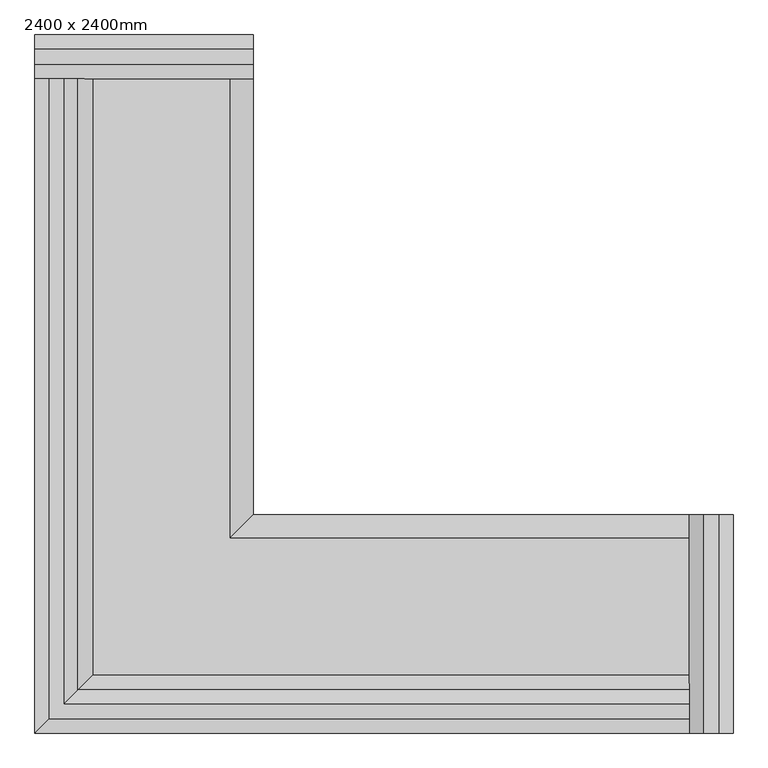
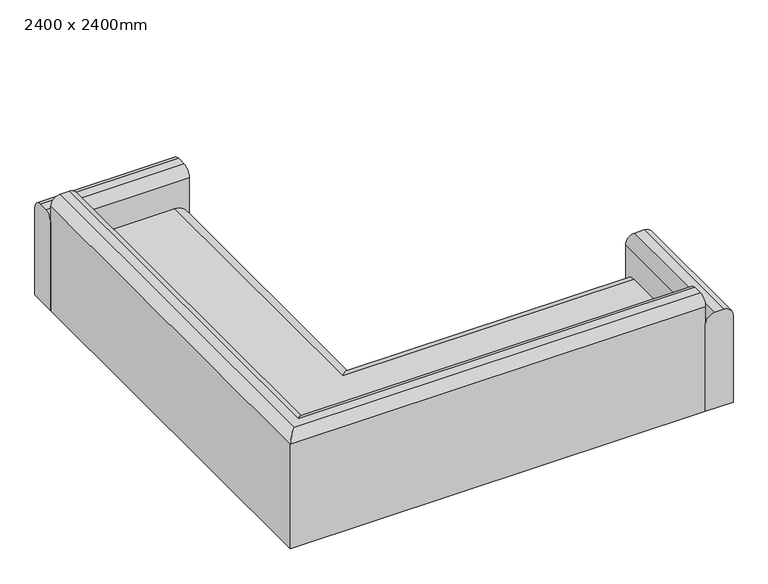
"""IFC4 building model written with IfcOpenShell, lengths in millimetres: furniture geometry, ソファ－L型 : 2400 x 2400mm."""

from ifc_helpers import new_model, si_unit, point, frame, frame_2d, origin, place, context, project, spatial, polyline, circle_curve, ellipse_curve, trimmed, segment, composite_curve, outline, extrude, source, transform, mapped, element, save
from ifc_brep_helpers import plane_surface, cylinder_surface, advanced_brep


def furniture_2400_x_2400mm_af02d185(model_context):
    return source(origin(), model_context, "Body", "SolidModel", [
        extrude(outline(composite_curve([segment(polyline([(1100.0, 550.0), (1150.0, 550.0)]), True, "CONTINUOUS"), segment(trimmed(circle_curve(frame_2d((1150.0, 500.0)), 50.0), [point((1150.0, 550.0))], [point((1200.0, 500.0))], False, "CARTESIAN"), True, "CONTINUOUS"), segment(polyline([(1200.0, 500.0), (1200.0, 0.0), (1050.0, 0.0), (1050.0, 500.0)]), True, "CONTINUOUS"), segment(trimmed(circle_curve(frame_2d((1100.0, 500.0)), 50.0), [point((1050.0, 500.0))], [point((1100.0, 550.0))], False, "CARTESIAN"), True, "CONTINUOUS")], self_intersect=False)), frame((-1200.0, 0.0, 0.0), z_axis=(1.0, 0.0, 0.0), x_axis=(0.0, 1.0, 0.0)), (0.0, 0.0, 1.0), 750.0),
        extrude(outline(composite_curve([segment(polyline([(550.0, 1150.0), (550.0, 1100.0)]), True, "CONTINUOUS"), segment(trimmed(circle_curve(frame_2d((500.0, 1100.0)), 50.0), [point((550.0, 1100.0))], [point((500.0, 1050.0))], False, "CARTESIAN"), True, "CONTINUOUS"), segment(polyline([(500.0, 1050.0), (0.0, 1050.0), (0.0, 1200.0), (500.0, 1200.0)]), True, "CONTINUOUS"), segment(trimmed(circle_curve(frame_2d((500.0, 1150.0)), 50.0), [point((500.0, 1200.0))], [point((550.0, 1150.0))], False, "CARTESIAN"), True, "CONTINUOUS")], self_intersect=False)), frame((0.0, -1200.0, 0.0), z_axis=(0.0, 1.0, 0.0), x_axis=(0.0, 0.0, 1.0)), (0.0, 0.0, 1.0), 750.0),
        advanced_brep(
        [(1050.0, -1150.0, 650.0), (1050.0, -1200.0, 600.0), (1050.0, -1200.0, 0.0), (1050.0, -490.0, 0.0), (1050.0, -490.0, 60.0), (1050.0, -450.0, 60.0), (1050.0, -450.0, 270.0), (1050.0, -530.0, 350.0), (1050.0, -1000.0, 350.0), (1050.0, -1051.9611614, 609.8058068), (1050.0, -1100.9901951, 650.0), (-1100.9901951, -1100.9901951, 650.0), (-1100.9901951, 1050.0, 650.0), (-1150.0, 1050.0, 650.0), (-1150.0, -1150.0, 650.0), (-1051.9611614, -1051.9611614, 609.8058068), (-1000.0, -1000.0, 350.0), (-530.0, -530.0, 350.0), (-530.0, 1050.0, 350.0), (-1000.0, 1050.0, 350.0), (-450.0, -450.0, 270.0), (-450.0, -450.0, 60.0), (-490.0, -490.0, 60.0), (-490.0, 1050.0, 60.0), (-450.0, 1050.0, 60.0), (-490.0, -490.0, 0.0), (-1200.0, -1200.0, 0.0), (-1200.0, 1050.0, 0.0), (-490.0, 1050.0, 0.0), (-1200.0, -1200.0, 600.0), (-1051.9611614, 1050.0, 609.8058068), (-450.0, 1050.0, 270.0), (-1200.0, 1050.0, 600.0)],
        [
            (0, 1, circle_curve(frame((1050.0, -1150.0, 600.0), z_axis=(1.0, 0.0, 0.0), x_axis=(0.0, 1.0, 0.0)), 50.0)),
            (1, 2),
            (2, 3),
            (3, 4),
            (4, 5),
            (5, 6),
            (6, 7, circle_curve(frame((1050.0, -530.0, 270.0), z_axis=(1.0, 0.0, 0.0), x_axis=(0.0, 1.0, 0.0)), 80.0)),
            (7, 8),
            (8, 9),
            (9, 10, circle_curve(frame((1050.0, -1100.9901951, 600.0), z_axis=(1.0, 0.0, 0.0), x_axis=(0.0, 1.0, 0.0)), 50.0)),
            (10, 0),
            (10, 11),
            (11, 12),
            (12, 13),
            (13, 14),
            (14, 0),
            (9, 15),
            (15, 11, ellipse_curve(frame((-1100.9901951, -1100.9901951, 600.0), z_axis=(0.7071067811865475, -0.7071067811865475, 0.0), x_axis=(0.7071067811865476, 0.7071067811865474, 0.0)), 70.7106781, 50.0)),
            (8, 16),
            (16, 15),
            (7, 17),
            (17, 18),
            (18, 19),
            (19, 16),
            (6, 20),
            (20, 17, ellipse_curve(frame((-530.0, -530.0, 270.0), z_axis=(0.7071067811865475, -0.7071067811865475, 0.0), x_axis=(0.7071067811865476, 0.7071067811865474, 0.0)), 113.137085, 80.0)),
            (5, 21),
            (21, 20),
            (4, 22),
            (22, 23),
            (23, 24),
            (24, 21),
            (3, 25),
            (25, 22),
            (2, 26),
            (26, 27),
            (27, 28),
            (28, 25),
            (1, 29),
            (29, 26),
            (14, 29, ellipse_curve(frame((-1150.0, -1150.0, 600.0), z_axis=(0.7071067811865475, -0.7071067811865475, 0.0), x_axis=(0.7071067811865476, 0.7071067811865474, 0.0)), 70.7106781, 50.0)),
            (12, 30, circle_curve(frame((-1100.9901951, 1050.0, 600.0), z_axis=(0.0, 1.0, 0.0), x_axis=(1.0, 0.0, 0.0)), 50.0)),
            (30, 19),
            (18, 31, circle_curve(frame((-530.0, 1050.0, 270.0), z_axis=(0.0, 1.0, 0.0), x_axis=(1.0, 0.0, 0.0)), 80.0)),
            (31, 24),
            (23, 28),
            (27, 32),
            (32, 13, circle_curve(frame((-1150.0, 1050.0, 600.0), z_axis=(0.0, 1.0, 0.0), x_axis=(1.0, 0.0, 0.0)), 50.0)),
            (15, 30),
            (20, 31),
            (29, 32),
        ],
        [
            plane_surface(frame((1050.0, -1200.0, -802.3539183), z_axis=(1.0, 0.0, 0.0), x_axis=(0.0, 1.0, 0.0))),
            plane_surface(frame((1050.0, -1150.0, 650.0), z_axis=(0.0, 0.0, 1.0), x_axis=(-1.0, 0.0, 0.0))),
            cylinder_surface(frame((1050.0, -1100.9901951, 600.0), z_axis=(1.0, 0.0, 0.0), x_axis=(0.0, 1.0, 0.0)), 50.0),
            plane_surface(frame((1050.0, -1051.9611614, 609.8058068), z_axis=(0.0, 0.9805806756909212, 0.19611613513817883), x_axis=(-1.0, 0.0, 0.0))),
            plane_surface(frame((1050.0, -1000.0, 350.0), z_axis=(0.0, 0.0, 1.0), x_axis=(-1.0, 0.0, 0.0))),
            cylinder_surface(frame((1050.0, -530.0, 270.0), z_axis=(1.0, 0.0, 0.0), x_axis=(0.0, 1.0, 0.0)), 80.0),
            plane_surface(frame((1050.0, -450.0, 270.0), z_axis=(0.0, 1.0, 0.0), x_axis=(-1.0, 0.0, 0.0))),
            plane_surface(frame((1050.0, -450.0, 60.0), z_axis=(0.0, 0.0, -1.0), x_axis=(-1.0, 0.0, 0.0))),
            plane_surface(frame((1050.0, -490.0, 60.0), z_axis=(0.0, 1.0, 0.0), x_axis=(-1.0, 0.0, 0.0))),
            plane_surface(frame((1050.0, -490.0, 0.0), z_axis=(0.0, 0.0, -1.0), x_axis=(-1.0, 0.0, 0.0))),
            plane_surface(frame((1050.0, -1200.0, 0.0), z_axis=(0.0, -1.0, 0.0), x_axis=(-1.0, 0.0, 0.0))),
            cylinder_surface(frame((1050.0, -1150.0, 600.0), z_axis=(1.0, 0.0, 0.0), x_axis=(0.0, 1.0, 0.0)), 50.0),
            plane_surface(frame((-2002.3539183, 1050.0, 0.0), z_axis=(0.0, 1.0, 0.0), x_axis=(0.0, 0.0, -1.0))),
            cylinder_surface(frame((-1100.9901951, -1200.0, 600.0), z_axis=(0.0, -1.0, 0.0), x_axis=(1.0, 0.0, 0.0)), 50.0),
            plane_surface(frame((-1051.9611614, -1051.9611614, 609.8058068), z_axis=(0.9805806756909212, 0.0, 0.19611613513817883), x_axis=(0.0, 1.0, 0.0))),
            cylinder_surface(frame((-530.0, -1200.0, 270.0), z_axis=(0.0, -1.0, 0.0), x_axis=(1.0, 0.0, 0.0)), 80.0),
            plane_surface(frame((-450.0, -450.0, 270.0), z_axis=(1.0, 0.0, 0.0), x_axis=(0.0, 1.0, 0.0))),
            plane_surface(frame((-490.0, -490.0, 60.0), z_axis=(1.0, 0.0, 0.0), x_axis=(0.0, 1.0, 0.0))),
            plane_surface(frame((-1200.0, -1200.0, 0.0), z_axis=(-1.0, 0.0, 0.0), x_axis=(0.0, 1.0, 0.0))),
            cylinder_surface(frame((-1150.0, -1200.0, 600.0), z_axis=(0.0, -1.0, 0.0), x_axis=(1.0, 0.0, 0.0)), 50.0),
        ],
        [
            (0, [[1, 2, 3, 4, 5, 6, 7, 8, 9, 10, 11]]),
            (1, [[12, 13, 14, 15, 16, -11]]),
            (2, [[17, 18, -12, -10]]),
            (3, [[19, 20, -17, -9]]),
            (4, [[21, 22, 23, 24, -19, -8]]),
            (5, [[25, 26, -21, -7]]),
            (6, [[27, 28, -25, -6]]),
            (7, [[29, 30, 31, 32, -27, -5]]),
            (8, [[33, 34, -29, -4]]),
            (9, [[35, 36, 37, 38, -33, -3]]),
            (10, [[39, 40, -35, -2]]),
            (11, [[-16, 41, -39, -1]]),
            (12, [[-14, 42, 43, -23, 44, 45, -31, 46, -37, 47, 48]]),
            (13, [[49, -42, -13, -18]]),
            (14, [[-24, -43, -49, -20]]),
            (15, [[50, -44, -22, -26]]),
            (16, [[-32, -45, -50, -28]]),
            (17, [[-38, -46, -30, -34]]),
            (18, [[51, -47, -36, -40]]),
            (19, [[-15, -48, -51, -41]]),
        ],
    ),
    ])


if __name__ == "__main__":
    model = new_model("IFC4")
    model_context = context("Model", 3, world=origin())
    ifc_project = project(units=[si_unit("LENGTHUNIT", "METRE", prefix="MILLI")], contexts=[model_context])
    site = spatial("IfcSite", under=ifc_project)
    building = spatial("IfcBuilding", under=site)
    placement = place(None, origin())
    furniture_2400_x_2400mm_shape = furniture_2400_x_2400mm_af02d185(model_context)
    element("IfcFurniture", 1, ObjectType="ソファ－L型 : 2400 x 2400mm", at=placement, inside=building, context=model_context, shape_type="MappedRepresentation", body=[
        mapped(furniture_2400_x_2400mm_shape, transform((0.0, 0.0, 0.0), x_axis=(1.0, 0.0, 0.0), y_axis=(0.0, 1.0, 0.0), z_axis=(0.0, 0.0, 1.0))),
    ])
    save(model, "model.ifc")

# Revit data of these elements
# Type "ソファ－L型 : 2400 x 2400mm"
#   Keynote = "12490.Y2"
#   座面高さ = 350 mm
#   幅 = 2400 mm
#   奥行き = 2400 mm
#   本体 = モチアミ - 無地 - グレー
#   Default Elevation = 0
# Element 1 (IfcFurniture, "ソファ－L型 : 2400 x 2400mm")
#   Materials on its faces: "モチアミ - 無地 - グレー"
# Materials
#   "モチアミ - 無地 - グレー": class "モチアミ", colour RGB 65 63 65, transparency 0, Cost = 0
